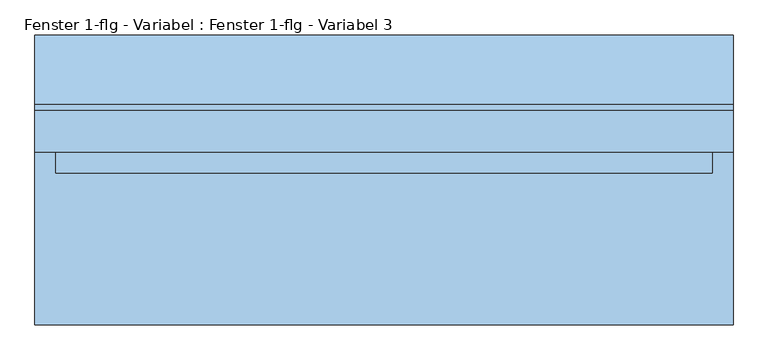
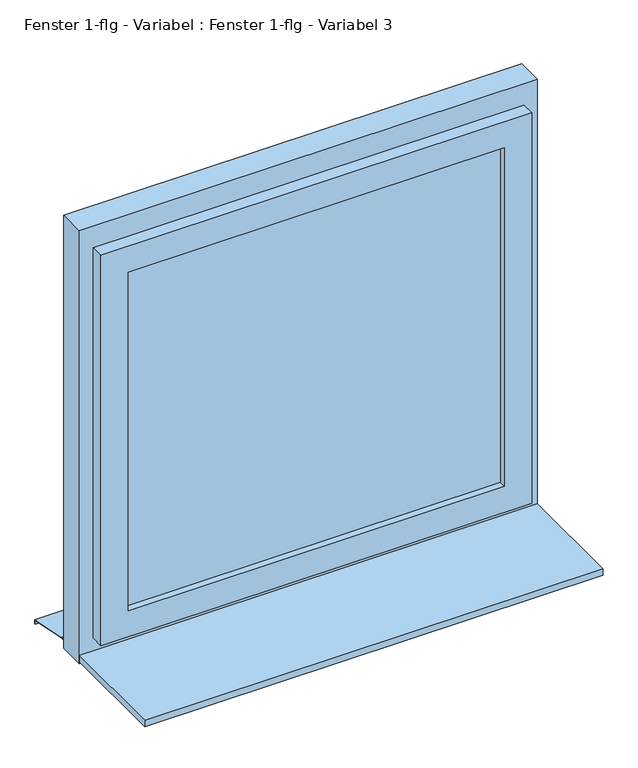
"""IFC4 building model written with IfcOpenShell, lengths in millimetres: window geometry, Fenster 1-flg - Variabel : Fenster 1-flg - Variabel 3."""

from ifc_helpers import new_model, si_unit, frame, origin, place, context, project, spatial, polyline, outline, extrude, faceted_brep, source, transform, mapped, element, save


def fenster_1_flg_variabel_fenster_1_flg_variabel_3_8a378bad(model_context):
    return source(origin(), model_context, "Body", "SolidModel", [
        extrude(outline(polyline([(2010.0, 505.0), (2010.0, -505.0), (1000.0, -505.0), (1000.0, 505.0), (2010.0, 505.0)]), holes=[polyline([(1930.0, 445.0), (1080.0, 445.0), (1080.0, -445.0), (1930.0, -445.0), (1930.0, 445.0)])]), frame((0.0, 40.0, 0.0), z_axis=(0.0, 1.0, 0.0), x_axis=(0.0, 0.0, 1.0)), (0.0, 0.0, 1.0), 60.0),
        faceted_brep([(475.0, 40.0, 1960.0), (475.0, 10.0, 1960.0), (475.0, 10.0, 1050.0), (475.0, 40.0, 1050.0), (-475.0, 10.0, 1960.0), (-475.0, 10.0, 1050.0), (415.0, 10.0, 1110.0), (-415.0, 10.0, 1110.0), (-415.0, 10.0, 1900.0), (415.0, 10.0, 1900.0), (-475.0, 40.0, 1050.0), (-475.0, 40.0, 1960.0), (445.0, 40.0, 1930.0), (-445.0, 40.0, 1930.0), (-445.0, 40.0, 1080.0), (445.0, 40.0, 1080.0), (445.0, 70.0, 1930.0), (445.0, 70.0, 1080.0), (-445.0, 70.0, 1080.0), (-445.0, 70.0, 1930.0), (415.0, 70.0, 1900.0), (-415.0, 70.0, 1900.0), (-415.0, 70.0, 1110.0), (415.0, 70.0, 1110.0)], [[[0, 1, 2, 3]], [[1, 4, 5, 2], [6, 7, 8, 9]], [[3, 2, 5, 10]], [[3, 10, 11, 0], [12, 13, 14, 15]], [[16, 12, 15, 17]], [[17, 15, 14, 18]], [[17, 18, 19, 16], [20, 21, 22, 23]], [[9, 20, 23, 6]], [[6, 23, 22, 7]], [[10, 5, 4, 11]], [[18, 14, 13, 19]], [[7, 22, 21, 8]], [[11, 4, 1, 0]], [[19, 13, 12, 16]], [[8, 21, 20, 9]]]),
        extrude(outline(polyline([(-505.0, -210.0), (-505.0, 40.0), (505.0, 40.0), (505.0, -210.0), (-505.0, -210.0)])), frame((0.0, 0.0, 1005.0), z_axis=(0.0, 0.0, 1.0), x_axis=(1.0, 0.0, 0.0)), (0.0, 0.0, 1.0), 15.0),
        extrude(outline(polyline([(110.0221543, 1020.0), (210.0, 1000.0), (210.0, 990.0), (208.0, 990.0), (208.0, 998.3604634), (109.8240723, 1018.0), (100.0, 1018.0), (100.0, 1020.0), (110.0221543, 1020.0)])), frame((-505.0, 0.0, 0.0), z_axis=(1.0, 0.0, 0.0), x_axis=(0.0, 1.0, 0.0)), (0.0, 0.0, 1.0), 1010.0),
        extrude(outline(polyline([(415.0, 25.0), (-415.0, 25.0), (-415.0, 55.0), (415.0, 55.0), (415.0, 25.0)])), frame((0.0, 0.0, 1110.0), z_axis=(0.0, 0.0, 1.0), x_axis=(1.0, 0.0, 0.0)), (0.0, 0.0, 1.0), 790.0),
    ])


if __name__ == "__main__":
    model = new_model("IFC4")
    model_context = context("Model", 3, world=origin())
    ifc_project = project(units=[si_unit("LENGTHUNIT", "METRE", prefix="MILLI")], contexts=[model_context])
    site = spatial("IfcSite", under=ifc_project)
    building = spatial("IfcBuilding", under=site)
    placement = place(None, origin())
    fenster_1_flg_variabel_fenster_1_flg_variabel_3_shape = fenster_1_flg_variabel_fenster_1_flg_variabel_3_8a378bad(model_context)
    element("IfcWindow", 1, ObjectType="Fenster 1-flg - Variabel : Fenster 1-flg - Variabel 3", at=placement, inside=building, context=model_context, shape_type="MappedRepresentation", body=[
        mapped(fenster_1_flg_variabel_fenster_1_flg_variabel_3_shape, transform((0.0, 0.0, 0.0), x_axis=(1.0, 0.0, 0.0), y_axis=(0.0, 1.0, 0.0), z_axis=(0.0, 0.0, 1.0))),
    ])
    save(model, "model.ifc")

# Revit data of these elements
# Type "Fenster 1-flg - Variabel : Fenster 1-flg - Variabel 3"
#   Type Mark = "52"
#   Operation = "SinglePanel"
#   Construction Type Id = "GSP4R"
#   Keynote = "16.05.01"
#   Analytic Construction = "1/8 Zoll Pilkington-Verglasung einfach"
#   Cost = 78.2
#   Visual Light Transmittance = 0.9
#   Höhe oberer  Rahmen = 0.080 m
#   Solar Heat Gain Coefficient = 0.86
#   Tiefe Flügel = 0.060 m
#   Rough Width [instance default] = 1.010 m
#   Rough Height [instance default] = 1.010 m
#   Rahmenhöhe unten = 0.080 m
#   Heat Transfer Coefficient (U) = 6.7069 W/(m²·K)
#   Rahmentiefe = 0.060 m
#   Rahmenbreite = 0.060 m
#   Height [instance default] = 1.010 m
#   Flügelbreite = 0.060 m
#   Einbautiefe (von außen) [instance default] = 0.080 m
#   Width [instance default] = 1.010 m
#   Define Thermal Properties by = 1
#   Öffnungsrichtung oben [instance default] = yes
#   Öffnungsrichtung in Draufsicht anzeigen [instance default] = no
#   Klappflügel [instance default] = no
#   Drehflügel 1 [instance default] = yes
#   Fensterflügel [instance default] = none
#   Innere Fensterbank [instance default] = none
#   Glas [instance default] = none
#   Bild [instance default] = none
#   Äußere Fensterbank [instance default] = none
#   Wall Closure = (empty or 0)
# Element 1 (IfcWindow, "Fenster 1-flg - Variabel : Fenster 1-flg - Variabel 3")
#   Materials on its faces: "Kunststoff - Weiß", "Holz - Birke", "Glas"
# Materials
#   "Kunststoff - Weiß": class "Kunststoff", colour RGB 249 249 249, transparency 0, Cost = 0
#   "Holz - Birke": class "Holz", colour RGB 213 164 103, transparency 0, Cost = 0
#   "Glas": class "Glas", colour RGB 0 0 255, transparency 0.75, Comments = "Render-Darstellung nicht aktualisiert ", Cost = 0
